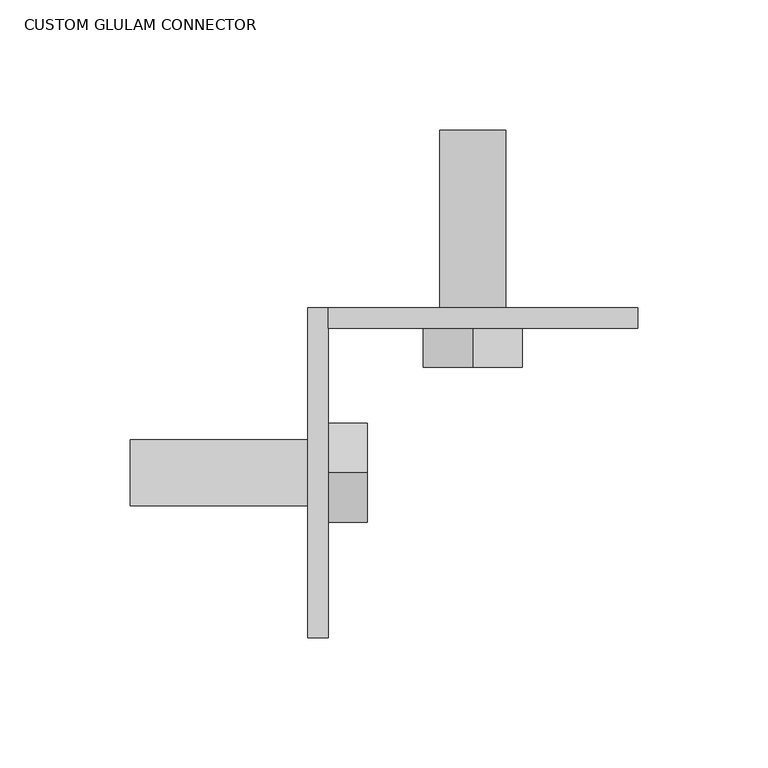
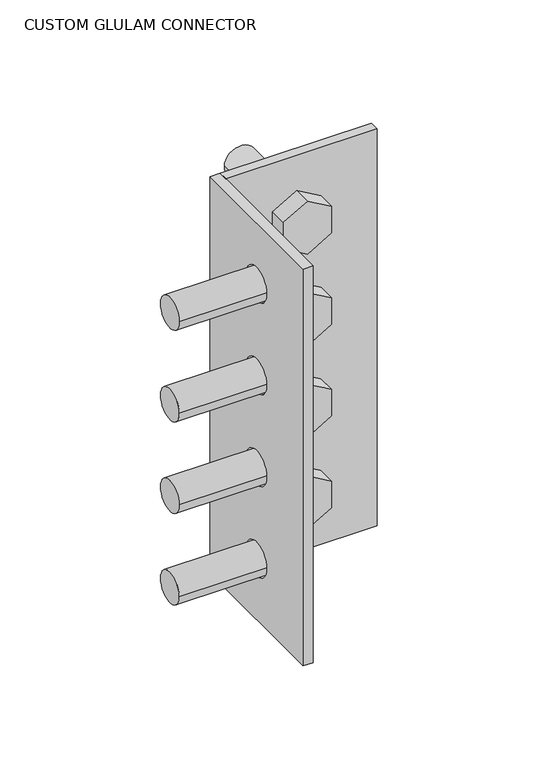
"""IFC4 building model written with IfcOpenShell, lengths in millimetres: fastener geometry, CUSTOM GLULAM CONNECTOR."""

import ifcopenshell
import ifcopenshell.guid

model = None  # the IFC model being written
_history = None  # IfcOwnerHistory: only IFC2X3 demands one
_inside = {}  # id of a spatial element -> (the spatial element, [elements in it])
_under = {}  # id of a project, library or spatial element -> (it, [spatial elements below it])
_declared = {}  # id of a project -> (the project, [libraries it declares])
_typed = {}  # id of a type object -> (the type object, [elements of that type])
_made_of = {}  # id of a material, layer set ... -> (it, [elements and type objects made of it])


def new_model(schema):
    """Start an empty IFC model of exactly this schema.

    Asked for "IFC4X3", IfcOpenShell would pick the latest addendum, in which some entities
    have other attributes; the version numbers below select the first issue.
    IFC2X3 requires an IfcOwnerHistory on every rooted entity: one is made here for all.
    """
    global model, _history
    if schema == "IFC4X3":
        model = ifcopenshell.file(schema_version=(4, 3, 0, 0))
    else:
        model = ifcopenshell.file(schema=schema)
    _inside.clear()
    _under.clear()
    _declared.clear()
    _typed.clear()
    _made_of.clear()
    _history = None
    if model.schema == "IFC2X3":
        org = make("IfcOrganization", Name="unknown")
        user = make(
            "IfcPersonAndOrganization",
            ThePerson=make("IfcPerson", FamilyName="unknown"),
            TheOrganization=org,
        )
        app = make(
            "IfcApplication",
            ApplicationDeveloper=org,
            Version="unknown",
            ApplicationFullName="unknown",
            ApplicationIdentifier="unknown",
        )
        _history = make(
            "IfcOwnerHistory",
            OwningUser=user,
            OwningApplication=app,
            ChangeAction="ADDED",
            CreationDate=0,
        )
    return model


def make(cls, **values):
    """One entity of the class cls with the attributes given. An attribute that is None is left unset."""
    return model.create_entity(
        cls, **{name: value for name, value in values.items() if value is not None}
    )


def rooted(cls, **values):
    """An entity with a GlobalId (a new one), such as an element, a storey or a relation."""
    return make(cls, GlobalId=ifcopenshell.guid.new(), OwnerHistory=_history, **values)


def si_unit(unit_type, name, prefix=None):
    """IfcSIUnit, for example si_unit("LENGTHUNIT", "METRE", prefix="MILLI")."""
    return make("IfcSIUnit", UnitType=unit_type, Prefix=prefix, Name=name)


def assignment(units):
    """IfcUnitAssignment: the units of a project."""
    return None if units is None else make("IfcUnitAssignment", Units=units)


def point(xyz):
    """IfcCartesianPoint."""
    return None if xyz is None else make("IfcCartesianPoint", Coordinates=xyz)


def direction(xyz):
    """IfcDirection."""
    return None if xyz is None else make("IfcDirection", DirectionRatios=xyz)


def frame(location, z_axis=None, x_axis=None):
    """IfcAxis2Placement3D, a coordinate frame: its origin and axes. An axis left out is left unset."""
    return make(
        "IfcAxis2Placement3D",
        Location=point(location),
        Axis=direction(z_axis),
        RefDirection=direction(x_axis),
    )


def frame_2d(location, x_axis=None):
    """IfcAxis2Placement2D, a coordinate frame in the plane: its origin and x axis."""
    return make(
        "IfcAxis2Placement2D", Location=point(location), RefDirection=direction(x_axis)
    )


def origin():
    """The frame at (0, 0, 0) with its axes left unset."""
    return frame((0.0, 0.0, 0.0))


def place(relative_to, where):
    """IfcLocalPlacement: puts the frame where relative to a parent placement (None: the world)."""
    return make(
        "IfcLocalPlacement", PlacementRelTo=relative_to, RelativePlacement=where
    )


def context(
    kind, dimensions, precision=None, world=None, true_north=None, identifier=None
):
    """IfcGeometricRepresentationContext, for example the 3D "Model" context."""
    return make(
        "IfcGeometricRepresentationContext",
        ContextIdentifier=identifier,
        ContextType=kind,
        CoordinateSpaceDimension=dimensions,
        Precision=precision,
        WorldCoordinateSystem=world,
        TrueNorth=true_north,
    )


def project(units=None, contexts=None):
    """IfcProject with its units and contexts."""
    return rooted(
        "IfcProject",
        Name="project",
        RepresentationContexts=contexts,
        UnitsInContext=assignment(units),
    )


def spatial(cls, under=None, at=None, **own):
    """A site, building, storey or space (cls), placed at a placement, below another one or the project."""
    s = rooted(cls, ObjectPlacement=at, **own)
    if under is not None:
        _under.setdefault(under.id(), (under, []))[1].append(s)
    return s


def polyline(points):
    """IfcPolyline through the points."""
    return make("IfcPolyline", Points=[point(p) for p in points])


def circle_curve(where, radius):
    """IfcCircle in the frame where."""
    return make("IfcCircle", Position=where, Radius=radius)


def trimmed(basis, trim1, trim2, sense, master):
    """IfcTrimmedCurve: the piece of a basis curve between two trims."""
    return make(
        "IfcTrimmedCurve",
        BasisCurve=basis,
        Trim1=trim1,
        Trim2=trim2,
        SenseAgreement=sense,
        MasterRepresentation=master,
    )


def segment(curve, same_sense, transition):
    """IfcCompositeCurveSegment."""
    return make(
        "IfcCompositeCurveSegment",
        Transition=transition,
        SameSense=same_sense,
        ParentCurve=curve,
    )


def composite_curve(segments, self_intersect=None):
    """IfcCompositeCurve: segments joined end to end."""
    return make("IfcCompositeCurve", Segments=segments, SelfIntersect=self_intersect)


def outline(outer, holes=None, kind="AREA"):
    """IfcArbitraryClosedProfileDef: a profile drawn as a closed curve; with holes, ...WithVoids."""
    if holes is None:
        return make("IfcArbitraryClosedProfileDef", ProfileType=kind, OuterCurve=outer)
    return make(
        "IfcArbitraryProfileDefWithVoids",
        ProfileType=kind,
        OuterCurve=outer,
        InnerCurves=holes,
    )


def extrude(swept, where, along, depth):
    """IfcExtrudedAreaSolid: the profile swept, set in the frame where, extruded along a direction by depth."""
    return make(
        "IfcExtrudedAreaSolid",
        SweptArea=swept,
        Position=where,
        ExtrudedDirection=direction(along),
        Depth=depth,
    )


def shape(context_of_items, identifier, shape_type, items):
    """IfcShapeRepresentation: the items that make up one representation, for example the "Body"."""
    return make(
        "IfcShapeRepresentation",
        ContextOfItems=context_of_items,
        RepresentationIdentifier=identifier,
        RepresentationType=shape_type,
        Items=items,
    )


def source(mapping_origin, context_of_items, identifier, shape_type, items):
    """IfcRepresentationMap: a shape defined once, which mapped items show again and again."""
    return make(
        "IfcRepresentationMap",
        MappingOrigin=mapping_origin,
        MappedRepresentation=shape(context_of_items, identifier, shape_type, items),
    )


def transform(
    local_origin,
    x_axis=None,
    y_axis=None,
    z_axis=None,
    scale=None,
    scale2=None,
    scale3=None,
    uniform=True,
):
    """IfcCartesianTransformationOperator3D, or its non-uniform kind. x_axis, y_axis, z_axis: its Axis1, 2, 3."""
    if uniform:
        return make(
            "IfcCartesianTransformationOperator3D",
            Axis1=direction(x_axis),
            Axis2=direction(y_axis),
            LocalOrigin=point(local_origin),
            Scale=scale,
            Axis3=direction(z_axis),
        )
    return make(
        "IfcCartesianTransformationOperator3DnonUniform",
        Axis1=direction(x_axis),
        Axis2=direction(y_axis),
        LocalOrigin=point(local_origin),
        Scale=scale,
        Axis3=direction(z_axis),
        Scale2=scale2,
        Scale3=scale3,
    )


def mapped(mapping_source, mapping_target):
    """IfcMappedItem: shows the shape of a source again, moved by a transform."""
    return make(
        "IfcMappedItem", MappingSource=mapping_source, MappingTarget=mapping_target
    )


def made_of(thing, what):
    """Note that an element or type object is made of a material, layer set ...; save() writes the relation."""
    if what is not None:
        _made_of.setdefault(what.id(), (what, []))[1].append(thing)
    return thing


def element(
    cls,
    number,
    at=None,
    inside=None,
    cuts=None,
    type_object=None,
    material=None,
    context=None,
    identifier="Body",
    shape_type=None,
    held_by="IfcProductDefinitionShape",
    body=None,
    shapes=None,
    **own,
):
    """One element of the class cls, such as IfcWall. Its Tag is "e" and its number.

    at: its placement. inside: the storey or other place that contains it. cuts: it is an
    opening in that element (IfcRelVoidsElement). A single representation is given by context,
    identifier, shape_type and body (its items); several are given by shapes. held_by: the class
    of the entity that holds the representations. save() writes the other relations.
    """
    e = rooted(cls, Tag="e%d" % number, ObjectPlacement=at, **own)
    if body is not None:
        shapes = [shape(context, identifier, shape_type, body)]
    if shapes is not None:
        e.Representation = make(held_by, Representations=shapes)
    if inside is not None:
        _inside.setdefault(inside.id(), (inside, []))[1].append(e)
    if cuts is not None:
        rooted(
            "IfcRelVoidsElement", RelatingBuildingElement=cuts, RelatedOpeningElement=e
        )
    if type_object is not None:
        _typed.setdefault(type_object.id(), (type_object, []))[1].append(e)
    return made_of(e, material)


def aggregate(whole, parts):
    """IfcRelAggregates: a whole, such as a stair, and the parts it consists of."""
    return rooted("IfcRelAggregates", RelatingObject=whole, RelatedObjects=parts)


def save(model, path):
    """Write the relations noted so far, then the file.

    IfcRelAggregates (storeys below a building ...), IfcRelContainedInSpatialStructure (elements
    in a storey), IfcRelDefinesByType, IfcRelAssociatesMaterial and IfcRelDeclares: one each for
    every whole, place, type object, material and project.
    """
    for whole, parts in _under.values():
        aggregate(whole, parts)
    for where, things in _inside.values():
        rooted(
            "IfcRelContainedInSpatialStructure",
            RelatedElements=things,
            RelatingStructure=where,
        )
    for kind, things in _typed.values():
        rooted("IfcRelDefinesByType", RelatedObjects=things, RelatingType=kind)
    for what, things in _made_of.values():
        rooted("IfcRelAssociatesMaterial", RelatedObjects=things, RelatingMaterial=what)
    for by, libraries in _declared.values():
        rooted("IfcRelDeclares", RelatingContext=by, RelatedDefinitions=libraries)
    model.write(path)


def plane_surface(at):
    """IfcPlane: the flat surface through the origin of the frame at, square to its z axis."""
    return make("IfcPlane", Position=at)


def revolved_surface(curve, axis_point, axis_direction):
    """IfcSurfaceOfRevolution: the curve turned about the line through axis_point along axis_direction."""
    return make(
        "IfcSurfaceOfRevolution",
        SweptCurve=make("IfcArbitraryOpenProfileDef", ProfileType="CURVE", Curve=curve),
        AxisPosition=make("IfcAxis1Placement", Location=point(axis_point), Axis=direction(axis_direction)),
    )


def advanced_brep(points, edges, surfaces, faces):
    """IfcAdvancedBrep: a solid bounded by faces that lie on surfaces and meet in shared edges.

    An edge is (start, end): straight between two places in points (the first is 0);
    or (start, end, curve); or (start, end, curve, False) where it runs against its curve.
    A face is (place in surfaces, loops), or (place, loops, False) where it looks against
    its surface's normal. A loop lists edges by number (the first is 1), with a minus sign
    where the edge is run from its end to its start. The first loop is the outer one.
    """
    corners = [point(p) for p in points]
    vertices = [make("IfcVertexPoint", VertexGeometry=c) for c in corners]
    made = []
    for start, end, *more in edges:
        made.append(
            make(
                "IfcEdgeCurve",
                EdgeStart=vertices[start],
                EdgeEnd=vertices[end],
                EdgeGeometry=more[0] if more else make("IfcPolyline", Points=[corners[start], corners[end]]),
                SameSense=more[1] if len(more) > 1 else True,
            )
        )
    hull = []
    for where, loops, *sense in faces:
        bounds = []
        for j, loop in enumerate(loops):
            ring = [make("IfcOrientedEdge", EdgeElement=made[abs(k) - 1], Orientation=k > 0) for k in loop]
            bounds.append(
                make(
                    "IfcFaceOuterBound" if j == 0 else "IfcFaceBound",
                    Bound=make("IfcEdgeLoop", EdgeList=ring),
                    Orientation=True,
                )
            )
        hull.append(make("IfcAdvancedFace", Bounds=bounds, FaceSurface=surfaces[where], SameSense=sense[0] if sense else True))
    return make("IfcAdvancedBrep", Outer=make("IfcClosedShell", CfsFaces=hull))


def custom_glulam_connector_0c2b97b1(model_context):
    return source(origin(), model_context, "Body", "SolidModel", [
        extrude(outline(polyline([(719.1375, 214.3125), (719.1375, 95.25), (388.9375, 95.25), (388.9375, 214.3125), (719.1375, 214.3125)]), holes=[composite_curve([segment(trimmed(circle_curve(frame_2d((668.3375, 150.8125)), 13.890625), [point((668.3375, 164.703125))], [point((668.3375, 136.921875))], True, "CARTESIAN"), True, "CONTINUOUS"), segment(trimmed(circle_curve(frame_2d((668.3375, 150.8125)), 13.890625), [point((668.3375, 136.921875))], [point((668.3375, 164.703125))], True, "CARTESIAN"), True, "CONTINUOUS")], self_intersect=False), composite_curve([segment(trimmed(circle_curve(frame_2d((592.1375, 150.8125)), 13.890625), [point((592.1375, 164.703125))], [point((592.1375, 136.921875))], True, "CARTESIAN"), True, "CONTINUOUS"), segment(trimmed(circle_curve(frame_2d((592.1375, 150.8125)), 13.890625), [point((592.1375, 136.921875))], [point((592.1375, 164.703125))], True, "CARTESIAN"), True, "CONTINUOUS")], self_intersect=False), composite_curve([segment(trimmed(circle_curve(frame_2d((515.9375, 150.8125)), 13.890625), [point((515.9375, 164.703125))], [point((515.9375, 136.921875))], True, "CARTESIAN"), True, "CONTINUOUS"), segment(trimmed(circle_curve(frame_2d((515.9375, 150.8125)), 13.890625), [point((515.9375, 136.921875))], [point((515.9375, 164.703125))], True, "CARTESIAN"), True, "CONTINUOUS")], self_intersect=False), composite_curve([segment(trimmed(circle_curve(frame_2d((439.7375, 150.8125)), 13.890625), [point((439.7375, 164.703125))], [point((439.7375, 136.921875))], True, "CARTESIAN"), True, "CONTINUOUS"), segment(trimmed(circle_curve(frame_2d((439.7375, 150.8125)), 13.890625), [point((439.7375, 136.921875))], [point((439.7375, 164.703125))], True, "CARTESIAN"), True, "CONTINUOUS")], self_intersect=False)]), frame((0.0, 55.5625, 0.0), z_axis=(0.0, 1.0, 0.0), x_axis=(0.0, 0.0, 1.0)), (0.0, 0.0, 1.0), 7.9375),
        extrude(outline(polyline([(679.3360226, 131.7625), (657.3389774, 131.7625), (646.3404547, 150.8125), (657.3389774, 169.8625), (679.3360226, 169.8625), (690.3345453, 150.8125), (679.3360226, 131.7625)])), frame((0.0, 40.5804688, 0.0), z_axis=(0.0, 1.0, 0.0), x_axis=(0.0, 0.0, 1.0)), (0.0, 0.0, 1.0), 14.9820312),
        extrude(outline(composite_curve([segment(trimmed(circle_curve(frame_2d((668.3375, 150.8125)), 12.7), [point((668.3375, 138.1125))], [point((668.3375, 163.5125))], False, "CARTESIAN"), True, "CONTINUOUS"), segment(trimmed(circle_curve(frame_2d((668.3375, 150.8125)), 12.7), [point((668.3375, 163.5125))], [point((668.3375, 138.1125))], False, "CARTESIAN"), True, "CONTINUOUS")], self_intersect=False)), frame((0.0, 55.5625, 0.0), z_axis=(0.0, 1.0, 0.0), x_axis=(0.0, 0.0, 1.0)), (0.0, 0.0, 1.0), 76.2),
        extrude(outline(polyline([(603.1360226, 131.7625), (581.1389774, 131.7625), (570.1404547, 150.8125), (581.1389774, 169.8625), (603.1360226, 169.8625), (614.1345453, 150.8125), (603.1360226, 131.7625)])), frame((0.0, 40.5804688, 0.0), z_axis=(0.0, 1.0, 0.0), x_axis=(0.0, 0.0, 1.0)), (0.0, 0.0, 1.0), 14.9820312),
        extrude(outline(composite_curve([segment(trimmed(circle_curve(frame_2d((592.1375, 150.8125)), 12.7), [point((592.1375, 138.1125))], [point((592.1375, 163.5125))], False, "CARTESIAN"), True, "CONTINUOUS"), segment(trimmed(circle_curve(frame_2d((592.1375, 150.8125)), 12.7), [point((592.1375, 163.5125))], [point((592.1375, 138.1125))], False, "CARTESIAN"), True, "CONTINUOUS")], self_intersect=False)), frame((0.0, 55.5625, 0.0), z_axis=(0.0, 1.0, 0.0), x_axis=(0.0, 0.0, 1.0)), (0.0, 0.0, 1.0), 76.2),
        extrude(outline(polyline([(679.3360226, 131.7625), (657.3389774, 131.7625), (646.3404547, 150.8125), (657.3389774, 169.8625), (679.3360226, 169.8625), (690.3345453, 150.8125), (679.3360226, 131.7625)])), frame((0.0, 40.5804688, 0.0), z_axis=(0.0, 1.0, 0.0), x_axis=(0.0, 0.0, 1.0)), (0.0, 0.0, 1.0), 14.9820312),
        extrude(outline(composite_curve([segment(trimmed(circle_curve(frame_2d((668.3375, 150.8125)), 12.7), [point((668.3375, 138.1125))], [point((668.3375, 163.5125))], False, "CARTESIAN"), True, "CONTINUOUS"), segment(trimmed(circle_curve(frame_2d((668.3375, 150.8125)), 12.7), [point((668.3375, 163.5125))], [point((668.3375, 138.1125))], False, "CARTESIAN"), True, "CONTINUOUS")], self_intersect=False)), frame((0.0, 55.5625, 0.0), z_axis=(0.0, 1.0, 0.0), x_axis=(0.0, 0.0, 1.0)), (0.0, 0.0, 1.0), 76.2),
        extrude(outline(polyline([(526.9360226, 131.7625), (504.9389774, 131.7625), (493.9404547, 150.8125), (504.9389774, 169.8625), (526.9360226, 169.8625), (537.9345453, 150.8125), (526.9360226, 131.7625)])), frame((0.0, 40.5804688, 0.0), z_axis=(0.0, 1.0, 0.0), x_axis=(0.0, 0.0, 1.0)), (0.0, 0.0, 1.0), 14.9820312),
        extrude(outline(composite_curve([segment(trimmed(circle_curve(frame_2d((515.9375, 150.8125)), 12.7), [point((515.9375, 138.1125))], [point((515.9375, 163.5125))], False, "CARTESIAN"), True, "CONTINUOUS"), segment(trimmed(circle_curve(frame_2d((515.9375, 150.8125)), 12.7), [point((515.9375, 163.5125))], [point((515.9375, 138.1125))], False, "CARTESIAN"), True, "CONTINUOUS")], self_intersect=False)), frame((0.0, 55.5625, 0.0), z_axis=(0.0, 1.0, 0.0), x_axis=(0.0, 0.0, 1.0)), (0.0, 0.0, 1.0), 76.2),
        extrude(outline(polyline([(450.7360226, 131.7625), (428.7389774, 131.7625), (417.7404547, 150.8125), (428.7389774, 169.8625), (450.7360226, 169.8625), (461.7345453, 150.8125), (450.7360226, 131.7625)])), frame((0.0, 40.5804688, 0.0), z_axis=(0.0, 1.0, 0.0), x_axis=(0.0, 0.0, 1.0)), (0.0, 0.0, 1.0), 14.9820312),
        extrude(outline(composite_curve([segment(trimmed(circle_curve(frame_2d((439.7375, 150.8125)), 12.7), [point((439.7375, 138.1125))], [point((439.7375, 163.5125))], False, "CARTESIAN"), True, "CONTINUOUS"), segment(trimmed(circle_curve(frame_2d((439.7375, 150.8125)), 12.7), [point((439.7375, 163.5125))], [point((439.7375, 138.1125))], False, "CARTESIAN"), True, "CONTINUOUS")], self_intersect=False)), frame((0.0, 55.5625, 0.0), z_axis=(0.0, 1.0, 0.0), x_axis=(0.0, 0.0, 1.0)), (0.0, 0.0, 1.0), 76.2),
        advanced_brep(
        [(95.25, 13.890625, 592.1375), (95.25, -13.890625, 592.1375), (87.3125, -13.890625, 592.1375), (87.3125, 13.890625, 592.1375), (95.25, 63.5, 719.1375), (87.3125, 63.5, 719.1375), (87.3125, -63.5, 719.1375), (95.25, -63.5, 719.1375), (95.25, 55.5625, 719.1375), (87.3125, 63.5, 388.9375), (87.3125, -63.5, 388.9375), (87.3125, 13.890625, 668.3375), (87.3125, -13.890625, 668.3375), (87.3125, 13.890625, 515.9375), (87.3125, -13.890625, 515.9375), (87.3125, 13.890625, 439.7375), (87.3125, -13.890625, 439.7375), (95.25, -63.5, 388.9375), (95.25, 55.5625, 388.9375), (95.25, 63.5, 388.9375), (95.25, -13.890625, 668.3375), (95.25, 13.890625, 668.3375), (95.25, -13.890625, 515.9375), (95.25, 13.890625, 515.9375), (95.25, -13.890625, 439.7375), (95.25, 13.890625, 439.7375)],
        [
            (0, 1, circle_curve(frame((95.25, 0.0, 592.1375), z_axis=(1.0, 0.0, 0.0), x_axis=(0.0, -1.0, 0.0)), 13.890625)),
            (1, 2),
            (2, 3, circle_curve(frame((87.3125, 0.0, 592.1375), z_axis=(-1.0, 0.0, 0.0), x_axis=(0.0, -1.0, 0.0)), 13.890625)),
            (3, 0),
            (4, 5),
            (5, 6),
            (6, 7),
            (7, 8),
            (8, 4),
            (5, 9),
            (9, 10),
            (10, 6),
            (11, 12, circle_curve(frame((87.3125, 0.0, 668.3375), z_axis=(1.0, 0.0, 0.0), x_axis=(0.0, -1.0, 0.0)), 13.890625)),
            (12, 11, circle_curve(frame((87.3125, 0.0, 668.3375), z_axis=(1.0, 0.0, 0.0), x_axis=(0.0, -1.0, 0.0)), 13.890625)),
            (2, 3, circle_curve(frame((87.3125, 0.0, 592.1375), z_axis=(1.0, 0.0, 0.0), x_axis=(0.0, -1.0, 0.0)), 13.890625)),
            (13, 14, circle_curve(frame((87.3125, 0.0, 515.9375), z_axis=(1.0, 0.0, 0.0), x_axis=(0.0, -1.0, 0.0)), 13.890625)),
            (14, 13, circle_curve(frame((87.3125, 0.0, 515.9375), z_axis=(1.0, 0.0, 0.0), x_axis=(0.0, -1.0, 0.0)), 13.890625)),
            (15, 16, circle_curve(frame((87.3125, 0.0, 439.7375), z_axis=(1.0, 0.0, 0.0), x_axis=(0.0, -1.0, 0.0)), 13.890625)),
            (16, 15, circle_curve(frame((87.3125, 0.0, 439.7375), z_axis=(1.0, 0.0, 0.0), x_axis=(0.0, -1.0, 0.0)), 13.890625)),
            (7, 17),
            (17, 18),
            (18, 19),
            (19, 4),
            (20, 21, circle_curve(frame((95.25, 0.0, 668.3375), z_axis=(-1.0, 0.0, 0.0), x_axis=(0.0, -1.0, 0.0)), 13.890625)),
            (21, 20, circle_curve(frame((95.25, 0.0, 668.3375), z_axis=(-1.0, 0.0, 0.0), x_axis=(0.0, -1.0, 0.0)), 13.890625)),
            (0, 1, circle_curve(frame((95.25, 0.0, 592.1375), z_axis=(-1.0, 0.0, 0.0), x_axis=(0.0, -1.0, 0.0)), 13.890625)),
            (22, 23, circle_curve(frame((95.25, 0.0, 515.9375), z_axis=(-1.0, 0.0, 0.0), x_axis=(0.0, -1.0, 0.0)), 13.890625)),
            (23, 22, circle_curve(frame((95.25, 0.0, 515.9375), z_axis=(-1.0, 0.0, 0.0), x_axis=(0.0, -1.0, 0.0)), 13.890625)),
            (24, 25, circle_curve(frame((95.25, 0.0, 439.7375), z_axis=(-1.0, 0.0, 0.0), x_axis=(0.0, -1.0, 0.0)), 13.890625)),
            (25, 24, circle_curve(frame((95.25, 0.0, 439.7375), z_axis=(-1.0, 0.0, 0.0), x_axis=(0.0, -1.0, 0.0)), 13.890625)),
            (19, 9),
            (10, 17),
            (12, 20),
            (21, 11),
            (22, 14),
            (13, 23),
            (24, 16),
            (15, 25),
        ],
        [
            revolved_surface(polyline([(95.25, -13.890625, 592.1375), (87.3125, -13.890625, 592.1375)]), (87.3125, 0.0, 592.1375), (1.0, 0.0, 0.0)),
            plane_surface(frame((95.25, -63.5, 719.1375), z_axis=(0.0, 0.0, 1.0), x_axis=(-1.0, 0.0, 0.0))),
            plane_surface(frame((87.3125, 63.5, 719.1375), z_axis=(-1.0, 0.0, 0.0), x_axis=(0.0, -1.0, 0.0))),
            plane_surface(frame((95.25, 63.5, 719.1375), z_axis=(1.0, 0.0, 0.0), x_axis=(0.0, 1.0, 0.0))),
            plane_surface(frame((95.25, 63.5, 719.1375), z_axis=(0.0, 1.0, 0.0), x_axis=(-1.0, 0.0, 0.0))),
            plane_surface(frame((95.25, -63.5, 388.9375), z_axis=(0.0, -1.0, 0.0), x_axis=(-1.0, 0.0, 0.0))),
            revolved_surface(polyline([(95.25, -13.890625, 668.3375), (87.3125, -13.890625, 668.3375)]), (87.3125, 0.0, 668.3375), (1.0, 0.0, 0.0)),
            plane_surface(frame((95.25, 63.5, 388.9375), z_axis=(0.0, 0.0, -1.0), x_axis=(-1.0, 0.0, 0.0))),
            revolved_surface(polyline([(95.25, -13.890625, 515.9375), (87.3125, -13.890625, 515.9375)]), (87.3125, 0.0, 515.9375), (1.0, 0.0, 0.0)),
            revolved_surface(polyline([(95.25, -13.890625, 439.7375), (87.3125, -13.890625, 439.7375)]), (87.3125, 0.0, 439.7375), (1.0, 0.0, 0.0)),
        ],
        [
            (0, [[1, 2, 3, 4]]),
            (1, [[5, 6, 7, 8, 9]]),
            (2, [[-6, 10, 11, 12], [13, 14], [-3, 15], [16, 17], [18, 19]]),
            (3, [[20, 21, 22, 23, -9, -8], [24, 25], [-1, 26], [27, 28], [29, 30]]),
            (4, [[31, -10, -5, -23]]),
            (5, [[-7, -12, 32, -20]]),
            (6, [[-14, 33, -25, 34]]),
            (6, [[-24, -33, -13, -34]]),
            (0, [[-15, -2, -26, -4]]),
            (7, [[-32, -11, -31, -22, -21]]),
            (8, [[-27, 35, -16, 36]]),
            (9, [[-29, 37, -18, 38]]),
            (9, [[-19, -37, -30, -38]]),
            (8, [[-17, -35, -28, -36]]),
        ],
    ),
        extrude(outline(polyline([(19.05, 679.3360226), (19.05, 657.3389774), (0.0, 646.3404547), (-19.05, 657.3389774), (-19.05, 679.3360226), (0.0, 690.3345453), (19.05, 679.3360226)])), frame((95.25, 0.0, 0.0), z_axis=(1.0, 0.0, 0.0), x_axis=(0.0, 1.0, 0.0)), (0.0, 0.0, 1.0), 14.9820312),
        extrude(outline(composite_curve([segment(trimmed(circle_curve(frame_2d((0.0, 668.3375)), 12.7), [point((12.7, 668.3375))], [point((-12.7, 668.3375))], False, "CARTESIAN"), True, "CONTINUOUS"), segment(trimmed(circle_curve(frame_2d((0.0, 668.3375)), 12.7), [point((-12.7, 668.3375))], [point((12.7, 668.3375))], False, "CARTESIAN"), True, "CONTINUOUS")], self_intersect=False)), frame((19.05, 0.0, 0.0), z_axis=(1.0, 0.0, 0.0), x_axis=(0.0, 1.0, 0.0)), (0.0, 0.0, 1.0), 76.2),
        extrude(outline(polyline([(19.05, 603.1360226), (19.05, 581.1389774), (0.0, 570.1404547), (-19.05, 581.1389774), (-19.05, 603.1360226), (0.0, 614.1345453), (19.05, 603.1360226)])), frame((95.25, 0.0, 0.0), z_axis=(1.0, 0.0, 0.0), x_axis=(0.0, 1.0, 0.0)), (0.0, 0.0, 1.0), 14.9820312),
        extrude(outline(composite_curve([segment(trimmed(circle_curve(frame_2d((0.0, 592.1375)), 12.7), [point((12.7, 592.1375))], [point((-12.7, 592.1375))], False, "CARTESIAN"), True, "CONTINUOUS"), segment(trimmed(circle_curve(frame_2d((0.0, 592.1375)), 12.7), [point((-12.7, 592.1375))], [point((12.7, 592.1375))], False, "CARTESIAN"), True, "CONTINUOUS")], self_intersect=False)), frame((19.05, 0.0, 0.0), z_axis=(1.0, 0.0, 0.0), x_axis=(0.0, 1.0, 0.0)), (0.0, 0.0, 1.0), 76.2),
        extrude(outline(polyline([(19.05, 679.3360226), (19.05, 657.3389774), (0.0, 646.3404547), (-19.05, 657.3389774), (-19.05, 679.3360226), (0.0, 690.3345453), (19.05, 679.3360226)])), frame((95.25, 0.0, 0.0), z_axis=(1.0, 0.0, 0.0), x_axis=(0.0, 1.0, 0.0)), (0.0, 0.0, 1.0), 14.9820312),
        extrude(outline(composite_curve([segment(trimmed(circle_curve(frame_2d((0.0, 668.3375)), 12.7), [point((12.7, 668.3375))], [point((-12.7, 668.3375))], False, "CARTESIAN"), True, "CONTINUOUS"), segment(trimmed(circle_curve(frame_2d((0.0, 668.3375)), 12.7), [point((-12.7, 668.3375))], [point((12.7, 668.3375))], False, "CARTESIAN"), True, "CONTINUOUS")], self_intersect=False)), frame((19.05, 0.0, 0.0), z_axis=(1.0, 0.0, 0.0), x_axis=(0.0, 1.0, 0.0)), (0.0, 0.0, 1.0), 76.2),
        extrude(outline(polyline([(19.05, 526.9360226), (19.05, 504.9389774), (0.0, 493.9404547), (-19.05, 504.9389774), (-19.05, 526.9360226), (0.0, 537.9345453), (19.05, 526.9360226)])), frame((95.25, 0.0, 0.0), z_axis=(1.0, 0.0, 0.0), x_axis=(0.0, 1.0, 0.0)), (0.0, 0.0, 1.0), 14.9820312),
        extrude(outline(composite_curve([segment(trimmed(circle_curve(frame_2d((0.0, 515.9375)), 12.7), [point((12.7, 515.9375))], [point((-12.7, 515.9375))], False, "CARTESIAN"), True, "CONTINUOUS"), segment(trimmed(circle_curve(frame_2d((0.0, 515.9375)), 12.7), [point((-12.7, 515.9375))], [point((12.7, 515.9375))], False, "CARTESIAN"), True, "CONTINUOUS")], self_intersect=False)), frame((19.05, 0.0, 0.0), z_axis=(1.0, 0.0, 0.0), x_axis=(0.0, 1.0, 0.0)), (0.0, 0.0, 1.0), 76.2),
        extrude(outline(polyline([(19.05, 450.7360226), (19.05, 428.7389774), (0.0, 417.7404547), (-19.05, 428.7389774), (-19.05, 450.7360226), (0.0, 461.7345453), (19.05, 450.7360226)])), frame((95.25, 0.0, 0.0), z_axis=(1.0, 0.0, 0.0), x_axis=(0.0, 1.0, 0.0)), (0.0, 0.0, 1.0), 14.9820312),
        extrude(outline(composite_curve([segment(trimmed(circle_curve(frame_2d((0.0, 439.7375)), 12.7), [point((12.7, 439.7375))], [point((-12.7, 439.7375))], False, "CARTESIAN"), True, "CONTINUOUS"), segment(trimmed(circle_curve(frame_2d((0.0, 439.7375)), 12.7), [point((-12.7, 439.7375))], [point((12.7, 439.7375))], False, "CARTESIAN"), True, "CONTINUOUS")], self_intersect=False)), frame((19.05, 0.0, 0.0), z_axis=(1.0, 0.0, 0.0), x_axis=(0.0, 1.0, 0.0)), (0.0, 0.0, 1.0), 76.2),
    ])


if __name__ == "__main__":
    model = new_model("IFC4")
    model_context = context("Model", 3, world=origin())
    ifc_project = project(units=[si_unit("LENGTHUNIT", "METRE", prefix="MILLI")], contexts=[model_context])
    site = spatial("IfcSite", under=ifc_project)
    building = spatial("IfcBuilding", under=site)
    placement = place(None, origin())
    custom_glulam_connector_shape = custom_glulam_connector_0c2b97b1(model_context)
    element("IfcFastener", 1, ObjectType="CUSTOM GLULAM CONNECTOR : CUSTOM - L5\"x5\"x5/16\"x13\" - HDG", at=placement, inside=building, context=model_context, shape_type="MappedRepresentation", body=[
        mapped(custom_glulam_connector_shape, transform((0.0, 0.0, 0.0), x_axis=(1.0, 0.0, 0.0), y_axis=(0.0, 1.0, 0.0), z_axis=(0.0, 0.0, 1.0))),
    ])
    save(model, "model.ifc")

# Revit data of these elements
# Project information
#   Project Issue Date = "Issue Date"
#   Project Status = "Project Status"
#   Client Name = "Owner"
#   Project Address = "640 West Main Street, Lake Geneva, WI 53147"
#   Project Name = "The Downtowner"
#   Project Number = "Project Number"
# Type "CUSTOM GLULAM CONNECTOR : CUSTOM - L5\"x5\"x5/16\"x13\" - HDG"
#   Width - Top = 0' - 6 7/8"
#   Top/Bottom Plate Thickness = 0' - 0 5/16"
#   Top/Bottom Plate - Width = 0' - 7 1/2"
#   Rod Radius = 0' - 0 1/2"
#   Rod Length [instance default] = 1' - 0"
#   Plate Thickness = 0' - 0 5/16"
#   Offset - Upper Plate 2 = 0' - 0"
#   Height of Plate = 1' - 3"
#   Width - Bottom = 0' - 6 7/8"
#   Plate Width = 0' - 5"
#   Bracket Width = 0' - 5 1/4"
#   Bracket Thickness = 0' - 0 5/8"
#   Bracket Offset in X = 0' - 3 3/4"
#   Bracket Offset in Y = 0' - 0 3/4"
#   Bracket Offset = 0' - 1 1/2"
#   Bracket Leg = 0' - 8"
#   Bracket Hole Radius - Up = 0' - 0 1/2"
#   Bracket Hole Radius - Down = 0' - 0 1/2"
#   Bracket Hole Offset = 0' - 2"
#   Beam Width = 0' - 7 3/8"
#   Angle 2 = 61.00°
#   Angle 1 = 151.00°
#   Top Plate Visible = no
#   Rod Visibility = no
#   Plate Visibility - Upper Right 2 = yes
#   Plate Visibility - Upper Right 1 = yes
#   Plate Visibility - Upper Left 2 = no
#   Plate Visibility - Upper Left 1 = no
#   Plate Visibility - Lower Right 2 = no
#   Plate Visibility - Lower Right 1 = no
#   Plate Visibility - Lower Left 2 = no
#   Plate Visibility - Lower Left 1 = no
#   Bracket Visibility = no
#   Bottom Plate Visible = no
#   Upper Plates - 2 = element 1868899
#   Upper Plates - 1 = element 1868901
#   Lower Plates = element 1746392
#   Bracket Material = L5"x5"x5/16" STEEL ANGLE (HDG AFTER FABRICATION)
#   URL = ""
# Element 1 (IfcFastener, "CUSTOM GLULAM CONNECTOR : CUSTOM - L5\"x5\"x5/16\"x13\" - HDG")
#   Materials on its faces: "1\" GALV. LAG BOLT (LENGTH = 1/2\" SHY OF GLULAM DEPTH) -  (GALV. THRU BOLT IF PLATE ON OPP. SIDE OF STRUCT MEMBER)", "L5\"x5\"x5/16\" STEEL ANGLE (HDG AFTER FABRICATION)"
# Materials
#   "L5\"x5\"x5/16\" STEEL ANGLE (HDG AFTER FABRICATION)": class "Generic", colour RGB 232 232 232, transparency 0, Cost = 0
#   "1\" GALV. LAG BOLT (LENGTH = 1/2\" SHY OF GLULAM DEPTH) -  (GALV. THRU BOLT IF PLATE ON OPP. SIDE OF STRUCT MEMBER)": class "Generic", colour RGB 120 120 120, transparency 0, Cost = 0
